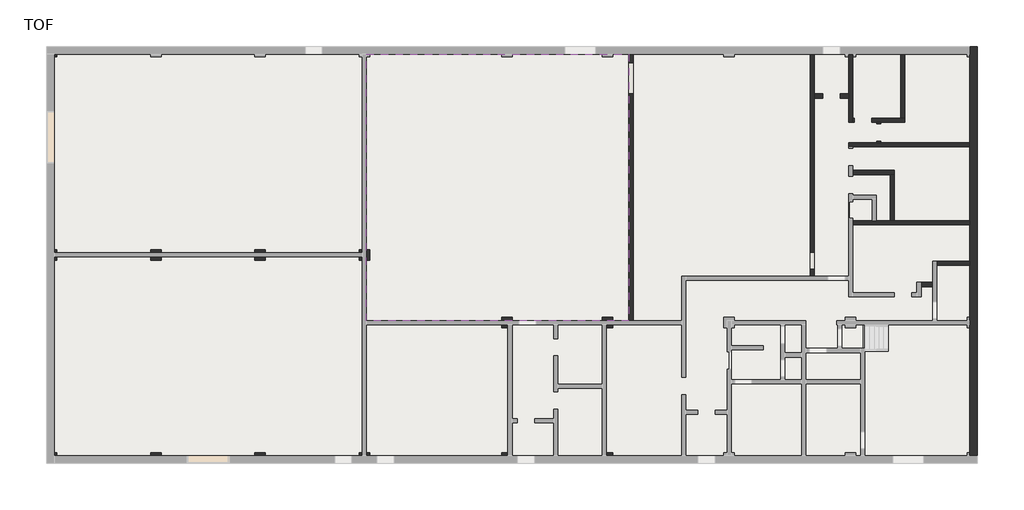
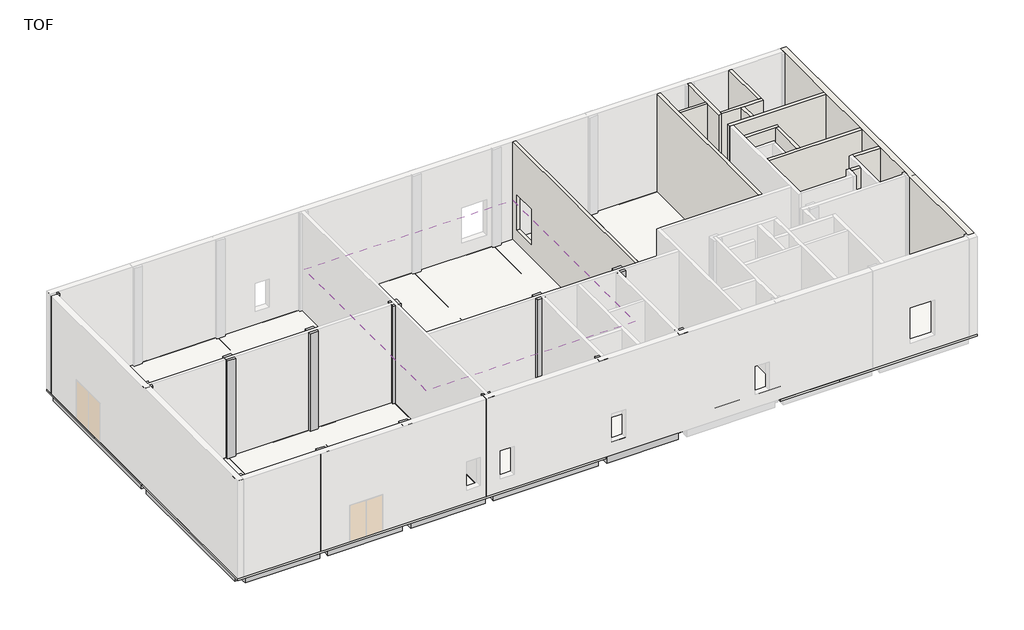
# One storey, part 2 of 3: 20 beams, 14 walls, 13 columns, 6 slabs, 1 covering.
"""IFC4 building model written with IfcOpenShell, lengths in millimetres."""

from ifc_helpers import new_model, si_unit, frame, origin, origin_with_axes, place, context, project, spatial, polyline, outline, extrude, faceted_brep, element, save

model = new_model("IFC4")

# Units and contexts
model_context = context("Model", 3, world=origin())
ifc_project = project(units=[si_unit("LENGTHUNIT", "METRE", prefix="MILLI")], contexts=[model_context])

# Site, building, storey
site = spatial("IfcSite", under=ifc_project)
building = spatial("IfcBuilding", under=site)
storey = spatial("IfcBuildingStorey", under=building, Name="TOF", Elevation=150.0)

# Beams
placement = place(None, origin())
element("IfcBeam", 1, ObjectType="RC Beam_Rectangular : H_SB_ACB_TG_B400xH600", at=placement, inside=storey, context=model_context, shape_type="SweptSolid", body=[
    extrude(outline(polyline([(99.7, 12616.5208589), (-250.3, 12616.5208589), (-250.3, 23716.5208589), (99.7, 23716.5208589), (99.7, 12616.5208589)])), frame((0.0, 0.0, -450.0), z_axis=(0.0, 0.0, 1.0), x_axis=(1.0, 0.0, 0.0)), (0.0, 0.0, 1.0), 600.0),
])
element("IfcBeam", 2, ObjectType="RC Beam_Rectangular : H_SB_ACB_TG_B400xH600", at=placement, inside=storey, context=model_context, shape_type="Brep", body=[
    faceted_brep([(99.7, 916.5208589, 150.0), (-250.3, 916.5208589, 150.0), (-250.3, 916.5208589, -450.0), (99.7, 916.5208589, -450.0), (-250.3, 12016.5208589, 150.0), (99.7, 12016.5208589, 150.0), (99.7, 12016.5208589, -450.0), (-250.3, 12016.5208589, -450.0), (99.7, 8241.5208589, 150.0), (99.7, 8591.5208589, 150.0), (99.7, 8591.5208589, -450.0), (99.7, 8241.5208589, -450.0)], [[[0, 1, 2, 3]], [[4, 5, 6, 7]], [[1, 0, 8, 9, 5, 4]], [[2, 1, 4, 7]], [[3, 2, 7, 6, 10, 11]], [[0, 3, 11, 10, 6, 5, 9, 8]]]),
])
element("IfcBeam", 3, ObjectType="RC Beam_Rectangular : H_SB_ACB_TG_B400xH600", at=placement, inside=storey, context=model_context, shape_type="SweptSolid", body=[
    extrude(outline(polyline([(224.7, 441.5208589), (224.7, 791.5208589), (5624.7, 791.5208589), (5624.7, 441.5208589), (224.7, 441.5208589)])), frame((0.0, 0.0, -450.0), z_axis=(0.0, 0.0, 1.0), x_axis=(1.0, 0.0, 0.0)), (0.0, 0.0, 1.0), 600.0),
])
element("IfcBeam", 4, ObjectType="RC Beam_Rectangular : H_SB_ACB_TG_B400xH600", at=placement, inside=storey, context=model_context, shape_type="SweptSolid", body=[
    extrude(outline(polyline([(6224.7, 441.5208589), (6224.7, 791.5208589), (11624.7, 791.5208589), (11624.7, 441.5208589), (6224.7, 441.5208589)])), frame((0.0, 0.0, -450.0), z_axis=(0.0, 0.0, 1.0), x_axis=(1.0, 0.0, 0.0)), (0.0, 0.0, 1.0), 600.0),
])
element("IfcBeam", 5, ObjectType="RC Beam_Rectangular : H_SB_ACB_TG_B400xH600", at=placement, inside=storey, context=model_context, shape_type="SweptSolid", body=[
    extrude(outline(polyline([(12224.7, 441.5208589), (12224.7, 791.5208589), (17624.7, 791.5208589), (17624.7, 441.5208589), (12224.7, 441.5208589)])), frame((0.0, 0.0, -450.0), z_axis=(0.0, 0.0, 1.0), x_axis=(1.0, 0.0, 0.0)), (0.0, 0.0, 1.0), 600.0),
])
element("IfcBeam", 6, ObjectType="RC Beam_Rectangular : H_SB_ACB_TG_B400xH600", at=placement, inside=storey, context=model_context, shape_type="SweptSolid", body=[
    extrude(outline(polyline([(18224.7, 441.5208589), (18224.7, 791.5208589), (25824.7, 791.5208589), (25824.7, 441.5208589), (18224.7, 441.5208589)])), frame((0.0, 0.0, -450.0), z_axis=(0.0, 0.0, 1.0), x_axis=(1.0, 0.0, 0.0)), (0.0, 0.0, 1.0), 600.0),
])
element("IfcBeam", 7, ObjectType="RC Beam_Rectangular : H_SB_ACB_TG_B400xH600", at=placement, inside=storey, context=model_context, shape_type="SweptSolid", body=[
    extrude(outline(polyline([(26424.7, 441.5208589), (26424.7, 791.5208589), (31624.7, 791.5208589), (31624.7, 441.5208589), (26424.7, 441.5208589)])), frame((0.0, 0.0, -450.0), z_axis=(0.0, 0.0, 1.0), x_axis=(1.0, 0.0, 0.0)), (0.0, 0.0, 1.0), 600.0),
])
element("IfcBeam", 8, ObjectType="RC Beam_Rectangular : H_SB_ACB_TG_B400xH600", at=placement, inside=storey, context=model_context, shape_type="Brep", body=[
    faceted_brep([(5749.7, 12016.5208589, 150.0), (6099.7, 12016.5208589, 150.0), (6099.7, 12016.5208589, -450.0), (5749.7, 12016.5208589, -450.0), (6099.7, 916.5208589, 150.0), (5749.7, 916.5208589, 150.0), (5749.7, 916.5208589, -450.0), (6099.7, 916.5208589, -450.0), (5749.7, 8591.5208589, 150.0), (5749.7, 8241.5208589, 150.0), (6099.7, 8241.5208589, 150.0), (6099.7, 8591.5208589, 150.0), (5749.7, 8591.5208589, -450.0), (5749.7, 8241.5208589, -450.0), (6099.7, 8591.5208589, -450.0), (6099.7, 8241.5208589, -450.0)], [[[0, 1, 2, 3]], [[4, 5, 6, 7]], [[1, 0, 8, 9, 5, 4, 10, 11]], [[0, 3, 12, 13, 6, 5, 9, 8]], [[3, 2, 14, 15, 7, 6, 13, 12]], [[2, 1, 11, 10, 4, 7, 15, 14]]]),
])
element("IfcBeam", 9, ObjectType="RC Beam_Rectangular : H_SB_ACB_TG_B400xH600", at=placement, inside=storey, context=model_context, shape_type="Brep", body=[
    faceted_brep([(11749.7, 12016.5208589, 150.0), (12099.7, 12016.5208589, 150.0), (12099.7, 12016.5208589, -450.0), (11749.7, 12016.5208589, -450.0), (12099.7, 916.5208589, 150.0), (11749.7, 916.5208589, 150.0), (11749.7, 916.5208589, -450.0), (12099.7, 916.5208589, -450.0), (11749.7, 8591.5208589, 150.0), (11749.7, 8241.5208589, 150.0), (12099.7, 8241.5208589, 150.0), (12099.7, 8591.5208589, 150.0), (11749.7, 8591.5208589, -450.0), (11749.7, 8241.5208589, -450.0), (12099.7, 8591.5208589, -450.0), (12099.7, 8241.5208589, -450.0)], [[[0, 1, 2, 3]], [[4, 5, 6, 7]], [[1, 0, 8, 9, 5, 4, 10, 11]], [[0, 3, 12, 13, 6, 5, 9, 8]], [[3, 2, 14, 15, 7, 6, 13, 12]], [[2, 1, 11, 10, 4, 7, 15, 14]]]),
])
element("IfcBeam", 10, ObjectType="RC Beam_Rectangular : H_SB_ACB_TG_B400xH600", at=placement, inside=storey, context=model_context, shape_type="Brep", body=[
    faceted_brep([(17749.7, 12016.5208589, 150.0), (18099.7, 12016.5208589, 150.0), (18099.7, 12016.5208589, -450.0), (17749.7, 12016.5208589, -450.0), (18099.7, 916.5208589, 150.0), (17749.7, 916.5208589, 150.0), (17749.7, 916.5208589, -450.0), (18099.7, 916.5208589, -450.0), (17749.7, 8591.5208589, 150.0), (17749.7, 8241.5208589, 150.0), (18099.7, 8241.5208589, 150.0), (18099.7, 8591.5208589, 150.0), (17749.7, 8591.5208589, -450.0), (17749.7, 8241.5208589, -450.0), (18099.7, 8591.5208589, -450.0), (18099.7, 8241.5208589, -450.0)], [[[0, 1, 2, 3]], [[4, 5, 6, 7]], [[1, 0, 8, 9, 5, 4, 10, 11]], [[0, 3, 12, 13, 6, 5, 9, 8]], [[3, 2, 14, 15, 7, 6, 13, 12]], [[2, 1, 11, 10, 4, 7, 15, 14]]]),
])
element("IfcBeam", 11, ObjectType="RC Beam_Rectangular : H_SB_ACB_TG_B400xH600", at=placement, inside=storey, context=model_context, shape_type="SweptSolid", body=[
    extrude(outline(polyline([(26299.7, 916.5208589), (25949.7, 916.5208589), (25949.7, 8116.5208589), (26299.7, 8116.5208589), (26299.7, 916.5208589)])), frame((0.0, 0.0, -450.0), z_axis=(0.0, 0.0, 1.0), x_axis=(1.0, 0.0, 0.0)), (0.0, 0.0, 1.0), 600.0),
])
element("IfcBeam", 12, ObjectType="RC Beam_Rectangular : H_SB_ACB_TG_B400xH600", at=placement, inside=storey, context=model_context, shape_type="SweptSolid", body=[
    extrude(outline(polyline([(224.7, 12141.5208589), (224.7, 12491.5208589), (5624.7, 12491.5208589), (5624.7, 12141.5208589), (224.7, 12141.5208589)])), frame((0.0, 0.0, -450.0), z_axis=(0.0, 0.0, 1.0), x_axis=(1.0, 0.0, 0.0)), (0.0, 0.0, 1.0), 600.0),
])
element("IfcBeam", 13, ObjectType="RC Beam_Rectangular : H_SB_ACB_TG_B400xH600", at=placement, inside=storey, context=model_context, shape_type="SweptSolid", body=[
    extrude(outline(polyline([(6224.7, 12141.5208589), (6224.7, 12491.5208589), (11624.7, 12491.5208589), (11624.7, 12141.5208589), (6224.7, 12141.5208589)])), frame((0.0, 0.0, -450.0), z_axis=(0.0, 0.0, 1.0), x_axis=(1.0, 0.0, 0.0)), (0.0, 0.0, 1.0), 600.0),
])
element("IfcBeam", 14, ObjectType="RC Beam_Rectangular : H_SB_ACB_TG_B400xH600", at=placement, inside=storey, context=model_context, shape_type="SweptSolid", body=[
    extrude(outline(polyline([(12224.7, 12141.5208589), (12224.7, 12491.5208589), (17624.7, 12491.5208589), (17624.7, 12141.5208589), (12224.7, 12141.5208589)])), frame((0.0, 0.0, -450.0), z_axis=(0.0, 0.0, 1.0), x_axis=(1.0, 0.0, 0.0)), (0.0, 0.0, 1.0), 600.0),
])
element("IfcBeam", 15, ObjectType="RC Beam_Rectangular : H_SB_ACB_TG_B400xH600", at=placement, inside=storey, context=model_context, shape_type="SweptSolid", body=[
    extrude(outline(polyline([(18224.7, 12141.5208589), (18224.7, 12491.5208589), (25949.7, 12491.5208589), (25949.7, 12141.5208589), (18224.7, 12141.5208589)])), frame((0.0, 0.0, -450.0), z_axis=(0.0, 0.0, 1.0), x_axis=(1.0, 0.0, 0.0)), (0.0, 0.0, 1.0), 600.0),
])
element("IfcBeam", 16, ObjectType="RC Beam_Rectangular : H_SB_ACB_TG_B400xH600", at=placement, inside=storey, context=model_context, shape_type="SweptSolid", body=[
    extrude(outline(polyline([(99.7, 8241.5208589), (99.7, 8591.5208589), (5749.7, 8591.5208589), (5749.7, 8241.5208589), (99.7, 8241.5208589)])), frame((0.0, 0.0, -450.0), z_axis=(0.0, 0.0, 1.0), x_axis=(1.0, 0.0, 0.0)), (0.0, 0.0, 1.0), 600.0),
])
element("IfcBeam", 17, ObjectType="RC Beam_Rectangular : H_SB_ACB_TG_B400xH600", at=placement, inside=storey, context=model_context, shape_type="SweptSolid", body=[
    extrude(outline(polyline([(6099.7, 8241.5208589), (6099.7, 8591.5208589), (11749.7, 8591.5208589), (11749.7, 8241.5208589), (6099.7, 8241.5208589)])), frame((0.0, 0.0, -450.0), z_axis=(0.0, 0.0, 1.0), x_axis=(1.0, 0.0, 0.0)), (0.0, 0.0, 1.0), 600.0),
])
element("IfcBeam", 18, ObjectType="RC Beam_Rectangular : H_SB_ACB_TG_B400xH600", at=placement, inside=storey, context=model_context, shape_type="SweptSolid", body=[
    extrude(outline(polyline([(12099.7, 8241.5208589), (12099.7, 8591.5208589), (17749.7, 8591.5208589), (17749.7, 8241.5208589), (12099.7, 8241.5208589)])), frame((0.0, 0.0, -450.0), z_axis=(0.0, 0.0, 1.0), x_axis=(1.0, 0.0, 0.0)), (0.0, 0.0, 1.0), 600.0),
])
element("IfcBeam", 19, ObjectType="RC Beam_Rectangular : H_SB_ACB_TG_B400xH600", at=placement, inside=storey, context=model_context, shape_type="SweptSolid", body=[
    extrude(outline(polyline([(18099.7, 8241.5208589), (18099.7, 8591.5208589), (25824.7, 8591.5208589), (25824.7, 8241.5208589), (18099.7, 8241.5208589)])), frame((0.0, 0.0, -450.0), z_axis=(0.0, 0.0, 1.0), x_axis=(1.0, 0.0, 0.0)), (0.0, 0.0, 1.0), 600.0),
])
element("IfcBeam", 20, ObjectType="RC Beam_Rectangular : H_SB_ACB_TG_B400xH600", at=placement, inside=storey, context=model_context, shape_type="SweptSolid", body=[
    extrude(outline(polyline([(26424.7, 8241.5208589), (26424.7, 8591.5208589), (31624.7, 8591.5208589), (31624.7, 8241.5208589), (26424.7, 8241.5208589)])), frame((0.0, 0.0, -450.0), z_axis=(0.0, 0.0, 1.0), x_axis=(1.0, 0.0, 0.0)), (0.0, 0.0, 1.0), 600.0),
])

# Columns
element("IfcColumn", 21, ObjectType="RC_Column_Rectangular : H_SC_ACC_W600xL600", at=placement, inside=storey, context=model_context, shape_type="Brep", body=[
    faceted_brep([(224.7, 12616.5208589, 150.0), (224.7, 12016.5208589, 150.0), (-375.3, 12016.5208589, 150.0), (-375.3, 12316.5208589, 150.0), (-375.3, 12616.5208589, 150.0), (224.7, 12616.5208589, 7650.0), (224.7, 12516.5208589, 7650.0), (224.7, 12116.5208589, 7650.0), (224.7, 12016.5208589, 7650.0), (124.7, 12016.5208589, 7650.0), (-275.3, 12016.5208589, 7650.0), (-375.3, 12016.5208589, 7650.0), (-375.3, 12616.5208589, 7650.0), (-275.3, 12616.5208589, 7650.0), (124.7, 12616.5208589, 7650.0)], [[[0, 1, 2, 3, 4]], [[5, 6, 7, 8, 1, 0]], [[8, 9, 10, 11, 2, 1]], [[11, 12, 4, 3, 2]], [[12, 13, 14, 5, 0, 4]], [[5, 14, 13, 12, 11, 10, 9, 8, 7, 6]]]),
])
element("IfcColumn", 22, ObjectType="RC_Column_Rectangular : H_SC_ACC_W600xL600", at=placement, inside=storey, context=model_context, shape_type="Brep", body=[
    faceted_brep([(6224.7, 12616.5208589, 150.0), (6224.7, 12016.5208589, 150.0), (5624.7, 12016.5208589, 150.0), (5624.7, 12616.5208589, 150.0), (6224.7, 12616.5208589, 7650.0), (6224.7, 12516.5208589, 7650.0), (6224.7, 12116.5208589, 7650.0), (6224.7, 12016.5208589, 7650.0), (6124.7, 12016.5208589, 7650.0), (5724.7, 12016.5208589, 7650.0), (5624.7, 12016.5208589, 7650.0), (5624.7, 12116.5208589, 7650.0), (5624.7, 12516.5208589, 7650.0), (5624.7, 12616.5208589, 7650.0), (5724.7, 12616.5208589, 7650.0), (6124.7, 12616.5208589, 7650.0)], [[[0, 1, 2, 3]], [[4, 5, 6, 7, 1, 0]], [[7, 8, 9, 10, 2, 1]], [[10, 11, 12, 13, 3, 2]], [[13, 14, 15, 4, 0, 3]], [[4, 15, 14, 13, 12, 11, 10, 9, 8, 7, 6, 5]]]),
])
element("IfcColumn", 23, ObjectType="RC_Column_Rectangular : H_SC_ACC_W600xL600", at=placement, inside=storey, context=model_context, shape_type="Brep", body=[
    faceted_brep([(12224.7, 12616.5208589, 150.0), (12224.7, 12016.5208589, 150.0), (11624.7, 12016.5208589, 150.0), (11624.7, 12616.5208589, 150.0), (12224.7, 12616.5208589, 7650.0), (12224.7, 12516.5208589, 7650.0), (12224.7, 12116.5208589, 7650.0), (12224.7, 12016.5208589, 7650.0), (12124.7, 12016.5208589, 7650.0), (11724.7, 12016.5208589, 7650.0), (11624.7, 12016.5208589, 7650.0), (11624.7, 12116.5208589, 7650.0), (11624.7, 12516.5208589, 7650.0), (11624.7, 12616.5208589, 7650.0), (11724.7, 12616.5208589, 7650.0), (12124.7, 12616.5208589, 7650.0)], [[[0, 1, 2, 3]], [[4, 5, 6, 7, 1, 0]], [[7, 8, 9, 10, 2, 1]], [[10, 11, 12, 13, 3, 2]], [[13, 14, 15, 4, 0, 3]], [[4, 15, 14, 13, 12, 11, 10, 9, 8, 7, 6, 5]]]),
])
element("IfcColumn", 24, ObjectType="RC_Column_Rectangular : H_SC_ACC_W600xL600", at=placement, inside=storey, context=model_context, shape_type="Brep", body=[
    faceted_brep([(18224.7, 12616.5208589, 150.0), (18224.7, 12016.5208589, 150.0), (17624.7, 12016.5208589, 150.0), (17624.7, 12616.5208589, 150.0), (18224.7, 12616.5208589, 7650.0), (18224.7, 12516.5208589, 7650.0), (18224.7, 12116.5208589, 7650.0), (18224.7, 12016.5208589, 7650.0), (18124.7, 12016.5208589, 7650.0), (17724.7, 12016.5208589, 7650.0), (17624.7, 12016.5208589, 7650.0), (17624.7, 12116.5208589, 7650.0), (17624.7, 12516.5208589, 7650.0), (17624.7, 12616.5208589, 7650.0), (17724.7, 12616.5208589, 7650.0), (18124.7, 12616.5208589, 7650.0)], [[[0, 1, 2, 3]], [[4, 5, 6, 7, 1, 0]], [[7, 8, 9, 10, 2, 1]], [[10, 11, 12, 13, 3, 2]], [[13, 14, 15, 4, 0, 3]], [[4, 15, 14, 13, 12, 11, 10, 9, 8, 7, 6, 5]]]),
])
element("IfcColumn", 25, ObjectType="RC_Column_Rectangular : H_SC_ACC_W600xL600", at=placement, inside=storey, context=model_context, shape_type="Brep", body=[
    faceted_brep([(224.7, 24316.5208589, 150.0), (224.7, 23716.5208589, 150.0), (-375.3, 23716.5208589, 150.0), (-375.3, 24316.5208589, 150.0), (224.7, 24316.5208589, 7650.0), (224.7, 24216.5208589, 7650.0), (224.7, 23816.5208589, 7650.0), (224.7, 23716.5208589, 7650.0), (124.7, 23716.5208589, 7650.0), (-275.3, 23716.5208589, 7650.0), (-375.3, 23716.5208589, 7650.0), (-375.3, 24316.5208589, 7650.0), (-275.3, 24316.5208589, 7650.0), (124.7, 24316.5208589, 7650.0)], [[[0, 1, 2, 3]], [[4, 5, 6, 7, 1, 0]], [[7, 8, 9, 10, 2, 1]], [[10, 11, 3, 2]], [[11, 12, 13, 4, 0, 3]], [[4, 13, 12, 11, 10, 9, 8, 7, 6, 5]]]),
])
element("IfcColumn", 26, ObjectType="RC_Column_Rectangular : H_SC_ACC_W600xL600", at=placement, inside=storey, context=model_context, shape_type="Brep", body=[
    faceted_brep([(26424.7, 8716.5208589, 150.0), (26424.7, 8116.5208589, 150.0), (25824.7, 8116.5208589, 150.0), (25824.7, 8716.5208589, 150.0), (26424.7, 8716.5208589, 7650.0), (26424.7, 8616.5208589, 7650.0), (26424.7, 8216.5208589, 7650.0), (26424.7, 8116.5208589, 7650.0), (26324.7, 8116.5208589, 7650.0), (25924.7, 8116.5208589, 7650.0), (25824.7, 8116.5208589, 7650.0), (25824.7, 8216.5208589, 7650.0), (25824.7, 8616.5208589, 7650.0), (25824.7, 8716.5208589, 7650.0), (25924.7, 8716.5208589, 7650.0), (26324.7, 8716.5208589, 7650.0)], [[[0, 1, 2, 3]], [[4, 5, 6, 7, 1, 0]], [[7, 8, 9, 10, 2, 1]], [[10, 11, 12, 13, 3, 2]], [[13, 14, 15, 4, 0, 3]], [[4, 15, 14, 13, 12, 11, 10, 9, 8, 7, 6, 5]]]),
])
element("IfcColumn", 27, ObjectType="RC_Column_Rectangular : H_SC_ACC_W600xL600", at=placement, inside=storey, context=model_context, shape_type="Brep", body=[
    faceted_brep([(32224.7, 8716.5208589, 150.0), (32224.7, 8116.5208589, 150.0), (31624.7, 8116.5208589, 150.0), (31624.7, 8716.5208589, 150.0), (32224.7, 8716.5208589, 7650.0), (32224.7, 8616.5208589, 7650.0), (32224.7, 8216.5208589, 7650.0), (32224.7, 8116.5208589, 7650.0), (32124.7, 8116.5208589, 7650.0), (31724.7, 8116.5208589, 7650.0), (31624.7, 8116.5208589, 7650.0), (31624.7, 8216.5208589, 7650.0), (31624.7, 8616.5208589, 7650.0), (31624.7, 8716.5208589, 7650.0), (31724.7, 8716.5208589, 7650.0), (32124.7, 8716.5208589, 7650.0)], [[[0, 1, 2, 3]], [[4, 5, 6, 7, 1, 0]], [[7, 8, 9, 10, 2, 1]], [[10, 11, 12, 13, 3, 2]], [[13, 14, 15, 4, 0, 3]], [[4, 15, 14, 13, 12, 11, 10, 9, 8, 7, 6, 5]]]),
])
element("IfcColumn", 28, ObjectType="RC_Column_Rectangular : H_SC_ACC_W600xL600", at=placement, inside=storey, context=model_context, shape_type="Brep", body=[
    faceted_brep([(224.7, 916.5208589, 150.0), (224.7, 316.5208589, 150.0), (-375.3, 316.5208589, 150.0), (-375.3, 916.5208589, 150.0), (224.7, 916.5208589, 7650.0), (224.7, 816.5208589, 7650.0), (224.7, 416.5208589, 7650.0), (224.7, 316.5208589, 7650.0), (-375.3, 316.5208589, 7650.0), (-375.3, 916.5208589, 7650.0), (-275.3, 916.5208589, 7650.0), (124.7, 916.5208589, 7650.0)], [[[0, 1, 2, 3]], [[4, 5, 6, 7, 1, 0]], [[7, 8, 2, 1]], [[8, 9, 3, 2]], [[9, 10, 11, 4, 0, 3]], [[4, 11, 10, 9, 8, 7, 6, 5]]]),
])
element("IfcColumn", 29, ObjectType="RC_Column_Rectangular : H_SC_ACC_W600xL600", at=placement, inside=storey, context=model_context, shape_type="Brep", body=[
    faceted_brep([(6224.7, 916.5208589, 150.0), (6224.7, 316.5208589, 150.0), (5624.7, 316.5208589, 150.0), (5624.7, 916.5208589, 150.0), (6224.7, 916.5208589, 7650.0), (6224.7, 816.5208589, 7650.0), (6224.7, 416.5208589, 7650.0), (6224.7, 316.5208589, 7650.0), (5624.7, 316.5208589, 7650.0), (5624.7, 416.5208589, 7650.0), (5624.7, 816.5208589, 7650.0), (5624.7, 916.5208589, 7650.0), (5724.7, 916.5208589, 7650.0), (6124.7, 916.5208589, 7650.0)], [[[0, 1, 2, 3]], [[4, 5, 6, 7, 1, 0]], [[7, 8, 2, 1]], [[8, 9, 10, 11, 3, 2]], [[11, 12, 13, 4, 0, 3]], [[4, 13, 12, 11, 10, 9, 8, 7, 6, 5]]]),
])
element("IfcColumn", 30, ObjectType="RC_Column_Rectangular : H_SC_ACC_W600xL600", at=placement, inside=storey, context=model_context, shape_type="Brep", body=[
    faceted_brep([(12224.7, 916.5208589, 150.0), (12224.7, 316.5208589, 150.0), (11624.7, 316.5208589, 150.0), (11624.7, 916.5208589, 150.0), (12224.7, 916.5208589, 7650.0), (12224.7, 816.5208589, 7650.0), (12224.7, 416.5208589, 7650.0), (12224.7, 316.5208589, 7650.0), (11624.7, 316.5208589, 7650.0), (11624.7, 416.5208589, 7650.0), (11624.7, 816.5208589, 7650.0), (11624.7, 916.5208589, 7650.0), (11724.7, 916.5208589, 7650.0), (12124.7, 916.5208589, 7650.0)], [[[0, 1, 2, 3]], [[4, 5, 6, 7, 1, 0]], [[7, 8, 2, 1]], [[8, 9, 10, 11, 3, 2]], [[11, 12, 13, 4, 0, 3]], [[4, 13, 12, 11, 10, 9, 8, 7, 6, 5]]]),
])
element("IfcColumn", 31, ObjectType="RC_Column_Rectangular : H_SC_ACC_W600xL600", at=placement, inside=storey, context=model_context, shape_type="Brep", body=[
    faceted_brep([(18224.7, 916.5208589, 150.0), (18224.7, 316.5208589, 150.0), (17624.7, 316.5208589, 150.0), (17624.7, 916.5208589, 150.0), (18224.7, 916.5208589, 7650.0), (18224.7, 816.5208589, 7650.0), (18224.7, 416.5208589, 7650.0), (18224.7, 316.5208589, 7650.0), (17624.7, 316.5208589, 7650.0), (17624.7, 416.5208589, 7650.0), (17624.7, 816.5208589, 7650.0), (17624.7, 916.5208589, 7650.0), (17724.7, 916.5208589, 7650.0), (18124.7, 916.5208589, 7650.0)], [[[0, 1, 2, 3]], [[4, 5, 6, 7, 1, 0]], [[7, 8, 2, 1]], [[8, 9, 10, 11, 3, 2]], [[11, 12, 13, 4, 0, 3]], [[4, 13, 12, 11, 10, 9, 8, 7, 6, 5]]]),
])
element("IfcColumn", 32, ObjectType="RC_Column_Rectangular : H_SC_ACC_W600xL600", at=placement, inside=storey, context=model_context, shape_type="Brep", body=[
    faceted_brep([(26424.7, 916.5208589, 150.0), (26424.7, 316.5208589, 150.0), (25824.7, 316.5208589, 150.0), (25824.7, 916.5208589, 150.0), (26424.7, 916.5208589, 7650.0), (26424.7, 816.5208589, 7650.0), (26424.7, 416.5208589, 7650.0), (26424.7, 316.5208589, 7650.0), (25824.7, 316.5208589, 7650.0), (25824.7, 416.5208589, 7650.0), (25824.7, 816.5208589, 7650.0), (25824.7, 916.5208589, 7650.0), (25924.7, 916.5208589, 7650.0), (26324.7, 916.5208589, 7650.0)], [[[0, 1, 2, 3]], [[4, 5, 6, 7, 1, 0]], [[7, 8, 2, 1]], [[8, 9, 10, 11, 3, 2]], [[11, 12, 13, 4, 0, 3]], [[4, 13, 12, 11, 10, 9, 8, 7, 6, 5]]]),
])
element("IfcColumn", 33, ObjectType="RC_Column_Rectangular : H_SC_ACC_W600xL600", at=placement, inside=storey, context=model_context, shape_type="Brep", body=[
    faceted_brep([(32224.7, 916.5208589, 150.0), (32224.7, 316.5208589, 150.0), (31624.7, 316.5208589, 150.0), (31624.7, 916.5208589, 150.0), (32224.7, 916.5208589, 7650.0), (32224.7, 816.5208589, 7650.0), (32224.7, 416.5208589, 7650.0), (32224.7, 316.5208589, 7650.0), (31624.7, 316.5208589, 7650.0), (31624.7, 416.5208589, 7650.0), (31624.7, 816.5208589, 7650.0), (31624.7, 916.5208589, 7650.0), (31724.7, 916.5208589, 7650.0), (32124.7, 916.5208589, 7650.0)], [[[0, 1, 2, 3]], [[4, 5, 6, 7, 1, 0]], [[7, 8, 2, 1]], [[8, 9, 10, 11, 3, 2]], [[11, 12, 13, 4, 0, 3]], [[4, 13, 12, 11, 10, 9, 8, 7, 6, 5]]]),
])

# Covering
element("IfcCovering", 34, ObjectType="CE741_Acoustic Tiled Ceiling System_600x600x9t_T_bar", at=placement, inside=storey, context=model_context, shape_type="SweptSolid", body=[
    extrude(outline(polyline([(18041.7, 8533.5208589), (18041.7, 23886.5208589), (33157.7, 23886.5208589), (33157.7, 8533.5208589), (18041.7, 8533.5208589)])), frame((0.0, 0.0, 3150.0), z_axis=(0.0, 0.0, 1.0), x_axis=(1.0, 0.0, 0.0)), (0.0, 0.0, 1.0), 9.0),
])

# Slabs
element("IfcSlab", 35, ObjectType="H_FL_AMF_RC Slab_T150", at=placement, inside=storey, context=model_context, shape_type="Brep", body=[
    faceted_brep([(-375.3, 24316.5208589, 0.0), (43724.7, 24316.5208589, 0.0), (43724.7, 10966.5208589, 0.0), (36324.7, 10966.5208589, 0.0), (36324.7, 8416.5208589, 0.0), (17924.7, 8416.5208589, 0.0), (17924.7, 12316.5208589, 0.0), (-375.3, 12316.5208589, 0.0), (-375.3, 24316.5208589, 150.0), (-375.3, 23716.5208589, 150.0), (-375.3, 12616.5208589, 150.0), (-375.3, 12316.5208589, 150.0), (17924.7, 12316.5208589, 150.0), (17924.7, 8416.5208589, 150.0), (36324.7, 8416.5208589, 150.0), (36324.7, 10966.5208589, 150.0), (43724.7, 10966.5208589, 150.0), (43724.7, 24316.5208589, 150.0), (39224.7, 24316.5208589, 150.0), (38624.7, 24316.5208589, 150.0), (32224.7, 24316.5208589, 150.0), (31624.7, 24316.5208589, 150.0), (26424.7, 24316.5208589, 150.0), (25824.7, 24316.5208589, 150.0), (18224.7, 24316.5208589, 150.0), (17624.7, 24316.5208589, 150.0), (12224.7, 24316.5208589, 150.0), (11624.7, 24316.5208589, 150.0), (6224.7, 24316.5208589, 150.0), (5624.7, 24316.5208589, 150.0), (224.7, 24316.5208589, 150.0)], [[[0, 1, 2, 3, 4, 5, 6, 7]], [[8, 9, 10, 11, 12, 13, 14, 15, 16, 17, 18, 19, 20, 21, 22, 23, 24, 25, 26, 27, 28, 29, 30]], [[0, 7, 11, 10, 9, 8]], [[1, 0, 8, 30, 29, 28, 27, 26, 25, 24, 23, 22, 21, 20, 19, 18, 17]], [[2, 1, 17, 16]], [[3, 2, 16, 15]], [[4, 3, 15, 14]], [[5, 4, 14, 13]], [[6, 5, 13, 12]], [[7, 6, 12, 11]]]),
])
element("IfcSlab", 36, ObjectType="H_FL_AMF_RC Slab_T150", at=placement, inside=storey, context=model_context, shape_type="Brep", body=[
    faceted_brep([(53224.7, 11850.5208589, 1000.0), (50777.7, 11850.5208589, 1000.0), (50777.7, 8416.5208589, 1000.0), (46624.7, 8416.5208589, 1000.0), (46624.7, 5013.5208589, 1000.0), (43341.7, 5013.5208589, 1000.0), (43224.7, 5013.5208589, 1000.0), (43224.7, 8299.5208589, 1000.0), (43224.7, 8416.5208589, 1000.0), (39041.7, 8416.5208589, 1000.0), (38924.7, 8416.5208589, 1000.0), (38924.7, 746.5208589, 1000.0), (38924.7, 316.5208589, 1000.0), (26307.7, 316.5208589, 1000.0), (26307.7, 8416.5208589, 1000.0), (36324.7, 8416.5208589, 1000.0), (36324.7, 10966.5208589, 1000.0), (43724.7, 10966.5208589, 1000.0), (43724.7, 24316.5208589, 1000.0), (53224.7, 24316.5208589, 1000.0), (53224.7, 11850.5208589, 1150.0), (53224.7, 24316.5208589, 1150.0), (43724.7, 24316.5208589, 1150.0), (43724.7, 10966.5208589, 1150.0), (36324.7, 10966.5208589, 1150.0), (36324.7, 8416.5208589, 1150.0), (26307.7, 8416.5208589, 1150.0), (26307.7, 316.5208589, 1150.0), (38924.7, 316.5208589, 1150.0), (38924.7, 746.5208589, 1150.0), (38924.7, 5746.5208589, 1150.0), (38924.7, 6746.5208589, 1150.0), (38924.7, 8416.5208589, 1150.0), (39041.7, 8416.5208589, 1150.0), (43224.7, 8416.5208589, 1150.0), (43224.7, 8299.5208589, 1150.0), (43224.7, 5013.5208589, 1150.0), (43341.7, 5013.5208589, 1150.0), (46624.7, 5013.5208589, 1150.0), (46624.7, 8416.5208589, 1150.0), (50777.7, 8416.5208589, 1150.0), (50777.7, 11850.5208589, 1150.0)], [[[0, 1, 2, 3, 4, 5, 6, 7, 8, 9, 10, 11, 12, 13, 14, 15, 16, 17, 18, 19]], [[20, 21, 22, 23, 24, 25, 26, 27, 28, 29, 30, 31, 32, 33, 34, 35, 36, 37, 38, 39, 40, 41]], [[13, 12, 28, 27]], [[19, 18, 22, 21]], [[0, 19, 21, 20]], [[1, 0, 20, 41]], [[2, 1, 41, 40]], [[3, 2, 40, 39]], [[4, 3, 39, 38]], [[6, 5, 4, 38, 37, 36]], [[8, 7, 6, 36, 35, 34]], [[10, 9, 8, 34, 33, 32]], [[12, 11, 10, 32, 31, 30, 29, 28]], [[14, 13, 27, 26]], [[15, 14, 26, 25]], [[16, 15, 25, 24]], [[17, 16, 24, 23]], [[18, 17, 23, 22]]]),
])
element("IfcSlab", 37, ObjectType="H_FL_AMF_RC Slab_T150", at=placement, inside=storey, context=model_context, shape_type="SweptSolid", body=[
    extrude(outline(polyline([(17924.7, 12316.5208589), (17924.7, 8416.5208589), (26307.7, 8416.5208589), (26307.7, 316.5208589), (-375.3, 316.5208589), (-375.3, 12316.5208589), (17924.7, 12316.5208589)])), origin_with_axes(), (0.0, 0.0, 1.0), 150.0),
])
element("IfcSlab", 38, ObjectType="H_FL_AMF_RC Slab_T150", at=placement, inside=storey, context=model_context, shape_type="SweptSolid", body=[
    extrude(outline(polyline([(53224.7, 11850.5208589), (53224.7, 8416.5208589), (50777.7, 8416.5208589), (50777.7, 11850.5208589), (53224.7, 11850.5208589)])), frame((0.0, 0.0, 1000.0), z_axis=(0.0, 0.0, 1.0), x_axis=(1.0, 0.0, 0.0)), (0.0, 0.0, 1.0), 150.0),
])
element("IfcSlab", 39, ObjectType="H_FL_AMF_RC Slab_T150", at=placement, inside=storey, context=model_context, shape_type="SweptSolid", body=[
    extrude(outline(polyline([(46624.7, 8416.5208589), (53224.7, 8416.5208589), (53224.7, 316.5208589), (43224.7, 316.5208589), (43224.7, 5018.5208589), (46624.7, 5018.5208589), (46624.7, 8416.5208589)])), origin_with_axes(), (0.0, 0.0, 1.0), 150.0),
])
element("IfcSlab", 40, ObjectType="H_FL_AMF_RC Slab_T150", at=placement, inside=storey, context=model_context, shape_type="SweptSolid", body=[
    extrude(outline(polyline([(38924.7, 316.5208589), (38924.7, 8416.5208589), (43224.7, 8416.5208589), (43224.7, 316.5208589), (38924.7, 316.5208589)])), origin_with_axes(), (0.0, 0.0, 1.0), 150.0),
])

# Walls
element("IfcWall", 41, ObjectType="H_WA_AMW_Brick Wall_Ext (0.5B_50_1.0B / Emulsion)", at=placement, inside=storey, context=model_context, shape_type="Brep", body=[
    faceted_brep([(52794.7, 24316.5208589, 150.0), (52794.7, 23886.5208589, 150.0), (52794.7, 8533.5208589, 150.0), (52794.7, 8299.5208589, 150.0), (52794.7, 746.5208589, 150.0), (52794.7, 746.5208589, 7650.0), (52794.7, 8299.5208589, 7650.0), (52794.7, 8533.5208589, 7650.0), (52794.7, 11733.5208589, 7650.0), (52794.7, 11967.5208589, 7650.0), (52794.7, 14049.5208589, 7650.0), (52794.7, 14283.5208589, 7650.0), (52794.7, 18549.5208589, 7650.0), (52794.7, 18783.5208589, 7650.0), (52794.7, 23886.5208589, 7650.0), (52794.7, 24316.5208589, 7650.0), (53224.7, 24316.5208589, 150.0), (53224.7, 24316.5208589, 7650.0), (53224.7, 746.5208589, 7650.0), (53224.7, 746.5208589, 150.0)], [[[0, 1, 2, 3, 4, 5, 6, 7, 8, 9, 10, 11, 12, 13, 14, 15]], [[16, 17, 18, 19]], [[4, 3, 2, 1, 0, 16, 19]], [[15, 14, 13, 12, 11, 10, 9, 8, 7, 6, 5, 18, 17]], [[0, 15, 17, 16]], [[5, 4, 19, 18]]]),
])
element("IfcWall", 42, ObjectType="H_WA_AMW_Block Wall_Int_T200 (Both Plaster_Emulsion)", at=placement, inside=storey, context=model_context, shape_type="SweptSolid", body=[
    extrude(outline(polyline([(23886.5208589, 150.0), (8533.5208589, 150.0), (8533.5208589, 7650.0), (23886.5208589, 7650.0), (23886.5208589, 150.0)]), holes=[polyline([(23386.5208589, 1150.0), (23386.5208589, 3850.0), (21586.5208589, 3850.0), (21586.5208589, 1150.0), (23386.5208589, 1150.0)])]), frame((33157.7, 0.0, 0.0), z_axis=(1.0, 0.0, 0.0), x_axis=(0.0, 1.0, 0.0)), (0.0, 0.0, 1.0), 234.0),
])
element("IfcWall", 43, ObjectType="H_WA_AMW_Block Wall_Int_T200 (Both Plaster_Emulsion)", at=placement, inside=storey, context=model_context, shape_type="Brep", body=[
    faceted_brep([(43841.7, 11083.5208589, 150.0), (43841.7, 23886.5208589, 150.0), (43841.7, 23886.5208589, 7650.0), (43841.7, 21586.5208589, 7650.0), (43841.7, 21352.5208589, 7650.0), (43841.7, 11083.5208589, 7650.0), (43841.7, 12483.5208589, 3300.0), (43841.7, 12483.5208589, 1150.0), (43841.7, 11483.5208589, 1150.0), (43841.7, 11483.5208589, 3300.0), (43607.7, 23886.5208589, 150.0), (43607.7, 11083.5208589, 150.0), (43607.7, 11083.5208589, 7650.0), (43607.7, 23886.5208589, 7650.0), (43607.7, 12483.5208589, 1150.0), (43607.7, 12483.5208589, 3300.0), (43607.7, 11483.5208589, 3300.0), (43607.7, 11483.5208589, 1150.0)], [[[0, 1, 2, 3, 4, 5], [6, 7, 8, 9]], [[10, 11, 12, 13], [14, 15, 16, 17]], [[1, 0, 11, 10]], [[5, 4, 3, 2, 13, 12]], [[2, 1, 10, 13]], [[0, 5, 12, 11]], [[14, 7, 6, 15]], [[15, 6, 9, 16]], [[16, 9, 8, 17]], [[7, 14, 17, 8]]]),
])
element("IfcWall", 44, ObjectType="H_WA_AMW_Block Wall_Int_T200 (Both Plaster_Emulsion)", at=placement, inside=storey, context=model_context, shape_type="SweptSolid", body=[
    extrude(outline(polyline([(7650.0, 45807.7), (7650.0, 43841.7), (1150.0, 43841.7), (1150.0, 44324.7), (3300.0, 44324.7), (3300.0, 45324.7), (1150.0, 45324.7), (1150.0, 45807.7), (7650.0, 45807.7)])), frame((0.0, 21352.5208589, 0.0), z_axis=(0.0, 1.0, 0.0), x_axis=(0.0, 0.0, 1.0)), (0.0, 0.0, 1.0), 234.0),
])
element("IfcWall", 45, ObjectType="H_WA_AMW_Block Wall_Int_T200 (Both Plaster_Emulsion)", at=placement, inside=storey, context=model_context, shape_type="Brep", body=[
    faceted_brep([(45807.7, 23886.5208589, 1150.0), (45807.7, 21586.5208589, 1150.0), (45807.7, 21352.5208589, 1150.0), (45807.7, 19949.5208589, 1150.0), (45807.7, 19949.5208589, 7650.0), (45807.7, 21352.5208589, 7650.0), (45807.7, 21586.5208589, 7650.0), (45807.7, 23886.5208589, 7650.0), (46041.7, 23886.5208589, 1150.0), (46041.7, 23886.5208589, 7650.0), (46041.7, 20183.5208589, 7650.0), (46041.7, 19949.5208589, 7650.0), (46041.7, 19949.5208589, 1150.0), (46041.7, 20183.5208589, 1150.0)], [[[0, 1, 2, 3, 4, 5, 6, 7]], [[8, 9, 10, 11, 12, 13]], [[3, 2, 1, 0, 8, 13, 12]], [[7, 6, 5, 4, 11, 10, 9]], [[0, 7, 9, 8]], [[4, 3, 12, 11]]]),
])
element("IfcWall", 46, ObjectType="H_WA_AMW_Block Wall_Int_T200 (Both Plaster_Emulsion)", at=placement, inside=storey, context=model_context, shape_type="SweptSolid", body=[
    extrude(outline(polyline([(52794.7, 11733.5208589), (50894.7, 11733.5208589), (50894.7, 11967.5208589), (52794.7, 11967.5208589), (52794.7, 11733.5208589)])), frame((0.0, 0.0, 1150.0), z_axis=(0.0, 0.0, 1.0), x_axis=(1.0, 0.0, 0.0)), (0.0, 0.0, 1.0), 6500.0),
])
element("IfcWall", 47, ObjectType="H_WA_AMW_Block Wall_Int_T200 (Both Plaster_Emulsion)", at=placement, inside=storey, context=model_context, shape_type="SweptSolid", body=[
    extrude(outline(polyline([(50660.7, 10499.5208589), (49977.7, 10499.5208589), (49977.7, 10733.5208589), (50660.7, 10733.5208589), (50660.7, 10499.5208589)])), frame((0.0, 0.0, 1150.0), z_axis=(0.0, 0.0, 1.0), x_axis=(1.0, 0.0, 0.0)), (0.0, 0.0, 1.0), 6500.0),
])
element("IfcWall", 48, ObjectType="H_WA_AMW_Block Wall_Int_T200 (Both Plaster_Emulsion)", at=placement, inside=storey, context=model_context, shape_type="Brep", body=[
    faceted_brep([(45807.7, 18549.5208589, 1150.0), (46041.7, 18549.5208589, 1150.0), (52794.7, 18549.5208589, 1150.0), (52794.7, 18549.5208589, 7650.0), (46041.7, 18549.5208589, 7650.0), (45807.7, 18549.5208589, 7650.0), (45807.7, 18783.5208589, 1150.0), (45807.7, 18783.5208589, 7650.0), (47424.7, 18783.5208589, 7650.0), (47658.7, 18783.5208589, 7650.0), (52794.7, 18783.5208589, 7650.0), (52794.7, 18783.5208589, 1150.0), (47658.7, 18783.5208589, 1150.0), (47424.7, 18783.5208589, 1150.0)], [[[0, 1, 2, 3, 4, 5]], [[6, 7, 8, 9, 10, 11, 12, 13]], [[2, 1, 0, 6, 13, 12, 11]], [[5, 4, 3, 10, 9, 8, 7]], [[3, 2, 11, 10]], [[0, 5, 7, 6]]]),
])
element("IfcWall", 49, ObjectType="H_WA_AMW_Block Wall_Int_T200 (Both Plaster_Emulsion)", at=placement, inside=storey, context=model_context, shape_type="Brep", body=[
    faceted_brep([(49041.7, 19949.5208589, 7650.0), (47658.7, 19949.5208589, 7650.0), (47424.7, 19949.5208589, 7650.0), (46041.7, 19949.5208589, 7650.0), (46041.7, 19949.5208589, 1150.0), (46141.7, 19949.5208589, 1150.0), (46141.7, 19949.5208589, 3300.0), (47141.7, 19949.5208589, 3300.0), (47141.7, 19949.5208589, 1150.0), (47424.7, 19949.5208589, 1150.0), (47658.7, 19949.5208589, 1150.0), (49041.7, 19949.5208589, 1150.0), (46041.7, 20183.5208589, 7650.0), (48807.7, 20183.5208589, 7650.0), (49041.7, 20183.5208589, 7650.0), (49041.7, 20183.5208589, 1150.0), (48807.7, 20183.5208589, 1150.0), (47141.7, 20183.5208589, 1150.0), (47141.7, 20183.5208589, 3300.0), (46141.7, 20183.5208589, 3300.0), (46141.7, 20183.5208589, 1150.0), (46041.7, 20183.5208589, 1150.0)], [[[0, 1, 2, 3, 4, 5, 6, 7, 8, 9, 10, 11]], [[12, 13, 14, 15, 16, 17, 18, 19, 20, 21]], [[15, 11, 10, 9, 8, 17, 16]], [[4, 21, 20, 5]], [[3, 2, 1, 0, 14, 13, 12]], [[0, 11, 15, 14]], [[4, 3, 12, 21]], [[7, 18, 17, 8]], [[18, 7, 6, 19]], [[19, 6, 5, 20]]]),
])
element("IfcWall", 50, ObjectType="H_WA_AMW_Block Wall_Int_T200 (Both Plaster_Emulsion)", at=placement, inside=storey, context=model_context, shape_type="SweptSolid", body=[
    extrude(outline(polyline([(48807.7, 20183.5208589), (48807.7, 23886.5208589), (49041.7, 23886.5208589), (49041.7, 20183.5208589), (48807.7, 20183.5208589)])), frame((0.0, 0.0, 1150.0), z_axis=(0.0, 0.0, 1.0), x_axis=(1.0, 0.0, 0.0)), (0.0, 0.0, 1.0), 6500.0),
])
element("IfcWall", 51, ObjectType="H_WA_AMW_Block Wall_Int_T200 (Both Plaster_Emulsion)", at=placement, inside=storey, context=model_context, shape_type="SweptSolid", body=[
    extrude(outline(polyline([(18783.5208589, 7650.0), (19949.5208589, 7650.0), (19949.5208589, 1150.0), (19866.5208589, 1150.0), (19866.5208589, 3300.0), (18866.5208589, 3300.0), (18866.5208589, 1150.0), (18783.5208589, 1150.0), (18783.5208589, 7650.0)])), frame((47424.7, 0.0, 0.0), z_axis=(1.0, 0.0, 0.0), x_axis=(0.0, 1.0, 0.0)), (0.0, 0.0, 1.0), 234.0),
])
element("IfcWall", 52, ObjectType="H_WA_AMW_Block Wall_Int_T200 (Both Plaster_Emulsion)", at=placement, inside=storey, context=model_context, shape_type="Brep", body=[
    faceted_brep([(46041.7, 14049.5208589, 1150.0), (52794.7, 14049.5208589, 1150.0), (52794.7, 14049.5208589, 7650.0), (46041.7, 14049.5208589, 7650.0), (46041.7, 14283.5208589, 1150.0), (46041.7, 14283.5208589, 7650.0), (47167.7, 14283.5208589, 7650.0), (47401.7, 14283.5208589, 7650.0), (48207.7, 14283.5208589, 7650.0), (48441.7, 14283.5208589, 7650.0), (52794.7, 14283.5208589, 7650.0), (52794.7, 14283.5208589, 1150.0), (48441.7, 14283.5208589, 1150.0), (48207.7, 14283.5208589, 1150.0), (47401.7, 14283.5208589, 1150.0), (47167.7, 14283.5208589, 1150.0)], [[[0, 1, 2, 3]], [[4, 5, 6, 7, 8, 9, 10, 11, 12, 13, 14, 15]], [[1, 0, 4, 15, 14, 13, 12, 11]], [[3, 2, 10, 9, 8, 7, 6, 5]], [[2, 1, 11, 10]], [[0, 3, 5, 4]]]),
])
element("IfcWall", 53, ObjectType="H_WA_AMW_Block Wall_Int_T200 (Both Plaster_Emulsion)", at=placement, inside=storey, context=model_context, shape_type="Brep", body=[
    faceted_brep([(46041.7, 16946.5208589, 1150.0), (48207.7, 16946.5208589, 1150.0), (48441.7, 16946.5208589, 1150.0), (48441.7, 16946.5208589, 7650.0), (48207.7, 16946.5208589, 7650.0), (46041.7, 16946.5208589, 7650.0), (46041.7, 17180.5208589, 1150.0), (46041.7, 17180.5208589, 7650.0), (48441.7, 17180.5208589, 7650.0), (48441.7, 17180.5208589, 1150.0)], [[[0, 1, 2, 3, 4, 5]], [[6, 7, 8, 9]], [[2, 1, 0, 6, 9]], [[5, 4, 3, 8, 7]], [[0, 5, 7, 6]], [[3, 2, 9, 8]]]),
])
element("IfcWall", 54, ObjectType="H_WA_AMW_Block Wall_Int_T200 (Both Plaster_Emulsion)", at=placement, inside=storey, context=model_context, shape_type="SweptSolid", body=[
    extrude(outline(polyline([(48207.7, 14283.5208589), (48207.7, 16946.5208589), (48441.7, 16946.5208589), (48441.7, 14283.5208589), (48207.7, 14283.5208589)])), frame((0.0, 0.0, 1150.0), z_axis=(0.0, 0.0, 1.0), x_axis=(1.0, 0.0, 0.0)), (0.0, 0.0, 1.0), 6500.0),
])

save(model, "model.ifc")

# Revit data of these elements
# Type "RC Beam_Rectangular : H_SB_ACB_TG_B400xH600"
#   중앙부 하부근 = ""
#   중앙부 상부근 = ""
#   중앙부 보조근 = ""
#   중앙부 늑근 = ""
#   외단부 하부근 = ""
#   외단부 상부근 = ""
#   외단부 보조근 = ""
#   외단부 늑근 = ""
#   부호 = "TG2"
#   내단부 하부근 = ""
#   내단부 상부근 = ""
#   내단부 보조근 = ""
#   내단부 늑근 = ""
#   ALL 하부근 = "3-D20"
#   ALL 상부근 = "4-D20"
#   ALL 보조근 = ""
#   ALL 늑근 = "2-D10 @120"
#   Width = 350.000 mm
#   Height = 600.000 mm
#   Length [instance default] = 1524.000 mm
#   b = 350.000 mm
#   h = 600.000 mm
#   hec_material3 [instance default] = none
#   hec_material2 [instance default] = none
#   hec_material1 [instance default] = none
#   Structural Material [instance default] = none
#   Assembly Code = ""
# Type "RC_Column_Rectangular : H_SC_ACC_W600xL600"
#   Width = 600.000 mm
#   Length = 600.000 mm
#   hec_material3 [instance default] = none
#   hec_material2 [instance default] = none
#   hec_material1 [instance default] = none
#   Structural Material [instance default] = none
#   Description = (empty or 0)
# Type "CE741_Acoustic Tiled Ceiling System_600x600x9t_T_bar"
#   built-in parameter 1002203 = 1 (stored number, unit not read)
#   built-in parameter 1002202 = 1 (stored number, unit not read)
#   Layers, outside or top first: 9.000 mm no material (function 4)
# Type "H_FL_AMF_RC Slab_T150"
#   Keynote = ""
#   Type Comments = ""
#   Description = ""
#   Function = 1
#   Layers, outside or top first: 150.000 mm no material (function 1)
# Type "H_WA_AMW_Brick Wall_Ext (0.5B_50_1.0B / Emulsion)"
#   Type Comments = ""
#   Layers, outside or top first: 0.000 mm no material (function 100); 20.000 mm no material (function 2); 115.000 mm no material (function 1); 50.000 mm no material (function 3); 0.000 mm no material (function 100); 230.000 mm no material (function 1); 15.000 mm no material (function 2); 0.000 mm no material (function 100); 0.000 mm no material (function 100)
# Type "H_WA_AMW_Block Wall_Int_T200 (Both Plaster_Emulsion)"
#   Type Comments = ""
#   Layers, outside or top first: 0.000 mm no material (function 100); 12.000 mm no material (function 2); 200.000 mm no material (function 1); 12.000 mm no material (function 2); 10.000 mm no material (function 5)
# Elements 1, 2, 3, 4, 5, 6, 7, 8, 9, 10, 11, 12, 13, 14, 15, 16, 17, 18, 19, 20 (IfcBeam, "RC Beam_Rectangular : H_SB_ACB_TG_B400xH600")
#   hec_material3 = none
#   hec_material2 = none
#   hec_material1 = none
#   Structural Material = none
#   Phase Created = New Construction
# Elements 21, 22, 23, 24, 25, 26, 27, 28, 29, 30, 31, 32, 33 (IfcColumn, "RC_Column_Rectangular : H_SC_ACC_W600xL600")
#   Comments = ""
#   hec_material3 = none
#   hec_material2 = none
#   hec_material1 = none
#   Structural Material = none
#   Phase Created = New Construction
# Element 34 (IfcCovering, "CE741_Acoustic Tiled Ceiling System_600x600x9t_T_bar")
#   Height Offset From Level = 3000.000 mm
#   Phase Created = New Construction
# Element 35 (IfcSlab, "H_FL_AMF_RC Slab_T150")
#   Height Offset From Level = 0.000 mm
#   Phase Created = New Construction
#   Materials on its faces: "Default Floor"
# Elements 36, 38 (IfcSlab, "H_FL_AMF_RC Slab_T150")
#   Height Offset From Level = 1000.000 mm
#   Phase Created = New Construction
#   Materials on its faces: "Default Floor"
# Element 37 (IfcSlab, "H_FL_AMF_RC Slab_T150")
#   built-in parameter 1001955 = 1.5708 (stored number, unit not read)
#   Height Offset From Level = 0.000 mm
#   Phase Created = New Construction
#   Materials on its faces: "Default Floor"
# Element 39 (IfcSlab, "H_FL_AMF_RC Slab_T150")
#   built-in parameter 1001955 = 3.14159 (stored number, unit not read)
#   Height Offset From Level = 0.000 mm
#   Phase Created = New Construction
#   Materials on its faces: "Default Floor"
# Element 40 (IfcSlab, "H_FL_AMF_RC Slab_T150")
#   built-in parameter 1001955 = -1.5708 (stored number, unit not read)
#   Height Offset From Level = 0.000 mm
#   Phase Created = New Construction
#   Materials on its faces: "Default Floor"
# Element 41 (IfcWall, "H_WA_AMW_Brick Wall_Ext (0.5B_50_1.0B / Emulsion)")
#   Mark = "EW4"
#   Wall Loca = "EXT"
#   Wall Style Name = "Concrete Wall+Insulation+Gypsum Board"
#   Wall Finish-In = "Acrylic Emulsion Paint on Gypsum Board"
#   Wall Base Material-2 = "Glass Wool (Fiberglass)"
#   Wall Base Material-3 = "Concrete Wall"
#   Wall Finish-Ex = "Acrylic Emulsion Paint on Fair Faced Concrete"
#   Top Offset = 0.000 mm
#   Base Offset = 0.000 mm
#   wall height = 7500.000 mm
#   Wall Style No = EW51-1
#   Phase Created = New Construction
#   Base Constraint = TOF
#   Top Constraint = TOC
#   Materials on its faces: "Default Wall"
# Element 42 (IfcWall, "H_WA_AMW_Block Wall_Int_T200 (Both Plaster_Emulsion)")
#   Mark = "W3"
#   Wall Loca = "INT"
#   Wall Style Name = "Block Wall"
#   Wall Ref. = ""
#   Wall Finish-In = "Acrylic Emulsion Paint on Cement Plaster"
#   Wall Base Material-1 = "Concrete Block"
#   Wall Base Material-2 = ""
#   Wall Base Material-3 = ""
#   Wall Finish-Ex = "Acrylic Emulsion Paint on Cement Plaster"
#   Top Offset = 0.000 mm
#   Base Offset = 0.000 mm
#   wall height = 7500.000 mm
#   Wall Style No = IW21
#   Phase Created = New Construction
#   Base Constraint = TOF
#   Top Constraint = TOC
#   Materials on its faces: "Default Wall"
# Element 43 (IfcWall, "H_WA_AMW_Block Wall_Int_T200 (Both Plaster_Emulsion)")
#   Mark = "W7"
#   Wall Loca = "INT"
#   Wall Style Name = "Block Wall"
#   Wall Ref. = ""
#   Wall Finish-In = "Acrylic Emulsion Paint on Cement Plaster"
#   Wall Base Material-1 = "Concrete Block"
#   Wall Base Material-2 = ""
#   Wall Base Material-3 = ""
#   Wall Finish-Ex = "Acrylic Emulsion Paint on Cement Plaster"
#   Top Offset = 0.000 mm
#   Base Offset = 0.000 mm
#   wall height = 7500.000 mm
#   Wall Style No = IW21
#   Phase Created = New Construction
#   Base Constraint = TOF
#   Top Constraint = TOC
#   Materials on its faces: "Default Wall"
# Element 44 (IfcWall, "H_WA_AMW_Block Wall_Int_T200 (Both Plaster_Emulsion)")
#   Mark = "W8"
#   Wall Loca = "INT"
#   Wall Style Name = "Block Wall"
#   Wall Ref. = ""
#   Wall Finish-In = "Acrylic Emulsion Paint on Cement Plaster"
#   Wall Base Material-1 = "Concrete Block"
#   Wall Base Material-2 = ""
#   Wall Base Material-3 = ""
#   Wall Finish-Ex = "Acrylic Emulsion Paint on Cement Plaster"
#   built-in parameter 1001111 = 1000.000 mm
#   Top Offset = 0.000 mm
#   Base Offset = 1000.000 mm
#   wall height = 6500.000 mm
#   Wall Style No = IW21
#   Phase Created = New Construction
#   Base Constraint = TOF
#   Top Constraint = TOC
#   Materials on its faces: "Default Wall"
# Element 45 (IfcWall, "H_WA_AMW_Block Wall_Int_T200 (Both Plaster_Emulsion)")
#   Mark = "W9"
#   Wall Loca = "INT"
#   Wall Style Name = "Block Wall"
#   Wall Ref. = ""
#   Wall Finish-In = "Acrylic Emulsion Paint on Cement Plaster"
#   Wall Base Material-1 = "Concrete Block"
#   Wall Base Material-2 = ""
#   Wall Base Material-3 = ""
#   Wall Finish-Ex = "Acrylic Emulsion Paint on Cement Plaster"
#   built-in parameter 1001111 = 1000.000 mm
#   Top Offset = 0.000 mm
#   Base Offset = 1000.000 mm
#   wall height = 6500.000 mm
#   Wall Style No = IW21
#   Phase Created = New Construction
#   Base Constraint = TOF
#   Top Constraint = TOC
#   Materials on its faces: "Default Wall"
# Element 46 (IfcWall, "H_WA_AMW_Block Wall_Int_T200 (Both Plaster_Emulsion)")
#   Mark = "W12"
#   Wall Loca = "INT"
#   Wall Style Name = "Block Wall"
#   Wall Ref. = ""
#   Wall Finish-In = "Acrylic Emulsion Paint on Cement Plaster"
#   Wall Base Material-1 = "Concrete Block"
#   Wall Base Material-2 = ""
#   Wall Base Material-3 = ""
#   Wall Finish-Ex = "Acrylic Emulsion Paint on Cement Plaster"
#   built-in parameter 1001111 = 1000.000 mm
#   Top Offset = 0.000 mm
#   Base Offset = 1000.000 mm
#   wall height = 6500.000 mm
#   Wall Style No = IW21
#   Phase Created = New Construction
#   Base Constraint = TOF
#   Top Constraint = TOC
#   Materials on its faces: "Default Wall"
# Element 47 (IfcWall, "H_WA_AMW_Block Wall_Int_T200 (Both Plaster_Emulsion)")
#   Mark = "W14"
#   Wall Loca = "INT"
#   Wall Style Name = "Block Wall"
#   Wall Ref. = ""
#   Wall Finish-In = "Acrylic Emulsion Paint on Cement Plaster"
#   Wall Base Material-1 = "Concrete Block"
#   Wall Base Material-2 = ""
#   Wall Base Material-3 = ""
#   Wall Finish-Ex = "Acrylic Emulsion Paint on Cement Plaster"
#   built-in parameter 1001111 = 1000.000 mm
#   Top Offset = 0.000 mm
#   Base Offset = 1000.000 mm
#   wall height = 6500.000 mm
#   Wall Style No = IW21
#   Phase Created = New Construction
#   Base Constraint = TOF
#   Top Constraint = TOC
#   Materials on its faces: "Default Wall"
# Element 48 (IfcWall, "H_WA_AMW_Block Wall_Int_T200 (Both Plaster_Emulsion)")
#   Mark = "W30"
#   Wall Loca = "INT"
#   Wall Style Name = "Block Wall"
#   Wall Ref. = ""
#   Wall Finish-In = "Acrylic Emulsion Paint on Cement Plaster"
#   Wall Base Material-1 = "Concrete Block"
#   Wall Base Material-2 = ""
#   Wall Base Material-3 = ""
#   Wall Finish-Ex = "Acrylic Emulsion Paint on Cement Plaster"
#   built-in parameter 1001111 = 1000.000 mm
#   Top Offset = 0.000 mm
#   Base Offset = 1000.000 mm
#   wall height = 6500.000 mm
#   Wall Style No = IW21
#   Phase Created = New Construction
#   Base Constraint = TOF
#   Top Constraint = TOC
#   Materials on its faces: "Default Wall"
# Element 49 (IfcWall, "H_WA_AMW_Block Wall_Int_T200 (Both Plaster_Emulsion)")
#   Mark = "W32"
#   Wall Loca = "INT"
#   Wall Style Name = "Block Wall"
#   Wall Ref. = ""
#   Wall Finish-In = "Acrylic Emulsion Paint on Cement Plaster"
#   Wall Base Material-1 = "Concrete Block"
#   Wall Base Material-2 = ""
#   Wall Base Material-3 = ""
#   Wall Finish-Ex = "Acrylic Emulsion Paint on Cement Plaster"
#   built-in parameter 1001111 = 1000.000 mm
#   Top Offset = 0.000 mm
#   Base Offset = 1000.000 mm
#   wall height = 6500.000 mm
#   Wall Style No = IW21
#   Phase Created = New Construction
#   Base Constraint = TOF
#   Top Constraint = TOC
#   Materials on its faces: "Default Wall"
# Element 50 (IfcWall, "H_WA_AMW_Block Wall_Int_T200 (Both Plaster_Emulsion)")
#   Mark = "W33"
#   Wall Loca = "INT"
#   Wall Style Name = "Block Wall"
#   Wall Ref. = ""
#   Wall Finish-In = "Acrylic Emulsion Paint on Cement Plaster"
#   Wall Base Material-1 = "Concrete Block"
#   Wall Base Material-2 = ""
#   Wall Base Material-3 = ""
#   Wall Finish-Ex = "Acrylic Emulsion Paint on Cement Plaster"
#   built-in parameter 1001111 = 1000.000 mm
#   Top Offset = 0.000 mm
#   Base Offset = 1000.000 mm
#   wall height = 6500.000 mm
#   Wall Style No = IW21
#   Phase Created = New Construction
#   Base Constraint = TOF
#   Top Constraint = TOC
#   Materials on its faces: "Default Wall"
# Element 51 (IfcWall, "H_WA_AMW_Block Wall_Int_T200 (Both Plaster_Emulsion)")
#   Mark = "W35"
#   Wall Loca = "INT"
#   Wall Style Name = "Block Wall"
#   Wall Ref. = ""
#   Wall Finish-In = "Acrylic Emulsion Paint on Cement Plaster"
#   Wall Base Material-1 = "Concrete Block"
#   Wall Base Material-2 = ""
#   Wall Base Material-3 = ""
#   Wall Finish-Ex = "Acrylic Emulsion Paint on Cement Plaster"
#   built-in parameter 1001111 = 1000.000 mm
#   Top Offset = 0.000 mm
#   Base Offset = 1000.000 mm
#   wall height = 6500.000 mm
#   Wall Style No = IW21
#   Phase Created = New Construction
#   Base Constraint = TOF
#   Top Constraint = TOC
#   Materials on its faces: "Default Wall"
# Element 52 (IfcWall, "H_WA_AMW_Block Wall_Int_T200 (Both Plaster_Emulsion)")
#   Mark = "W36"
#   Wall Loca = "INT"
#   Wall Style Name = "Block Wall"
#   Wall Ref. = ""
#   Wall Finish-In = "Acrylic Emulsion Paint on Cement Plaster"
#   Wall Base Material-1 = "Concrete Block"
#   Wall Base Material-2 = ""
#   Wall Base Material-3 = ""
#   Wall Finish-Ex = "Acrylic Emulsion Paint on Cement Plaster"
#   built-in parameter 1001111 = 1000.000 mm
#   Top Offset = 0.000 mm
#   Base Offset = 1000.000 mm
#   wall height = 6500.000 mm
#   Wall Style No = IW21
#   Phase Created = New Construction
#   Base Constraint = TOF
#   Top Constraint = TOC
#   Materials on its faces: "Default Wall"
# Element 53 (IfcWall, "H_WA_AMW_Block Wall_Int_T200 (Both Plaster_Emulsion)")
#   Mark = "W37"
#   Wall Loca = "INT"
#   Wall Style Name = "Block Wall"
#   Wall Ref. = ""
#   Wall Finish-In = "Acrylic Emulsion Paint on Cement Plaster"
#   Wall Base Material-1 = "Concrete Block"
#   Wall Base Material-2 = ""
#   Wall Base Material-3 = ""
#   Wall Finish-Ex = "Acrylic Emulsion Paint on Cement Plaster"
#   built-in parameter 1001111 = 1000.000 mm
#   Top Offset = 0.000 mm
#   Base Offset = 1000.000 mm
#   wall height = 6500.000 mm
#   Wall Style No = IW21
#   Phase Created = New Construction
#   Base Constraint = TOF
#   Top Constraint = TOC
#   Materials on its faces: "Default Wall"
# Element 54 (IfcWall, "H_WA_AMW_Block Wall_Int_T200 (Both Plaster_Emulsion)")
#   Mark = "W38"
#   Wall Loca = "INT"
#   Wall Style Name = "Block Wall"
#   Wall Ref. = ""
#   Wall Finish-In = "Acrylic Emulsion Paint on Cement Plaster"
#   Wall Base Material-1 = "Concrete Block"
#   Wall Base Material-2 = ""
#   Wall Base Material-3 = ""
#   Wall Finish-Ex = "Acrylic Emulsion Paint on Cement Plaster"
#   built-in parameter 1001111 = 1000.000 mm
#   Top Offset = 0.000 mm
#   Base Offset = 1000.000 mm
#   wall height = 6500.000 mm
#   Wall Style No = IW21
#   Phase Created = New Construction
#   Base Constraint = TOF
#   Top Constraint = TOC
#   Materials on its faces: "Default Wall"
# Materials
#   "Default Floor": class "Miscellaneous", colour RGB 80 80 80, transparency 0
#   "Default Wall": class "Miscellaneous", colour RGB 80 80 80, transparency 0
